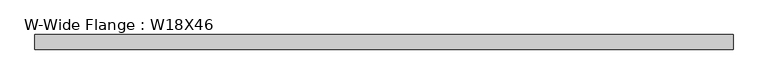
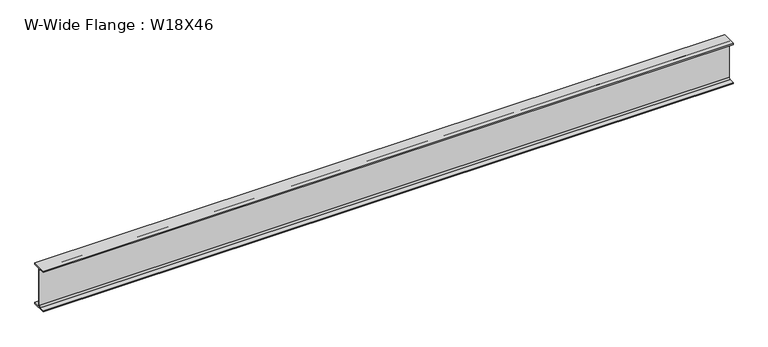
"""IFC4 building model written with IfcOpenShell, lengths in millimetres: beam geometry, W-Wide Flange : W18X46."""

from ifc_helpers import new_model, si_unit, point, frame, frame_2d, origin, place, context, project, spatial, polyline, circle_curve, trimmed, segment, composite_curve, outline, extrude, source, transform, mapped, element, save


def w_wide_flange_w18x46_b0132ec0(model_context):
    return source(origin(), model_context, "Body", "SweptSolid", [
        extrude(outline(composite_curve([segment(polyline([(76.962, -214.503), (76.962, -229.87), (-76.962, -229.87), (-76.962, -214.503), (-20.955, -214.503)]), True, "CONTINUOUS"), segment(trimmed(circle_curve(frame_2d((-20.955, -198.12)), 16.383), [point((-20.955, -214.503))], [point((-4.572, -198.12))], True, "CARTESIAN"), True, "CONTINUOUS"), segment(polyline([(-4.572, -198.12), (-4.572, 198.12)]), True, "CONTINUOUS"), segment(trimmed(circle_curve(frame_2d((-20.955, 198.12)), 16.383), [point((-4.572, 198.12))], [point((-20.955, 214.503))], True, "CARTESIAN"), True, "CONTINUOUS"), segment(polyline([(-20.955, 214.503), (-76.962, 214.503), (-76.962, 229.87), (76.962, 229.87), (76.962, 214.503), (20.955, 214.503)]), True, "CONTINUOUS"), segment(trimmed(circle_curve(frame_2d((20.955, 198.12)), 16.383), [point((20.955, 214.503))], [point((4.572, 198.12))], True, "CARTESIAN"), True, "CONTINUOUS"), segment(polyline([(4.572, 198.12), (4.572, -198.12)]), True, "CONTINUOUS"), segment(trimmed(circle_curve(frame_2d((20.955, -198.12)), 16.383), [point((4.572, -198.12))], [point((20.955, -214.503))], True, "CARTESIAN"), True, "CONTINUOUS"), segment(polyline([(20.955, -214.503), (76.962, -214.503)]), True, "CONTINUOUS")], self_intersect=False)), frame((-3648.0253906, 0.0, 0.0), z_axis=(1.0, 0.0, 0.0), x_axis=(0.0, 1.0, 0.0)), (0.0, 0.0, 1.0), 7358.7570312),
    ])


if __name__ == "__main__":
    model = new_model("IFC4")
    model_context = context("Model", 3, world=origin())
    ifc_project = project(units=[si_unit("LENGTHUNIT", "METRE", prefix="MILLI")], contexts=[model_context])
    site = spatial("IfcSite", under=ifc_project)
    building = spatial("IfcBuilding", under=site)
    placement = place(None, origin())
    w_wide_flange_w18x46_shape = w_wide_flange_w18x46_b0132ec0(model_context)
    element("IfcBeam", 1, ObjectType="W-Wide Flange : W18X46", at=placement, inside=building, context=model_context, shape_type="MappedRepresentation", body=[
        mapped(w_wide_flange_w18x46_shape, transform((0.0, 0.0, 0.0), x_axis=(1.0, 0.0, 0.0), y_axis=(0.0, 1.0, 0.0), z_axis=(0.0, 0.0, 1.0))),
    ])
    save(model, "model.ifc")

# Revit data of these elements
# Type "W-Wide Flange : W18X46"
#   Assembly Code = "B10"
#   W = 46
#   Length [instance default] = 1524 mm
#   bf = 153.924 mm
#   d = 459.74 mm
#   k = 31.75 mm
#   k2 = 16.383 mm
#   tf = 15.367 mm
#   tw = 9.144 mm
#   A = 0.00870966 m²
#   Structural Material [instance default] = Steel ASTM A992
# Element 1 (IfcBeam, "W-Wide Flange : W18X46")
#   Structural Material = Aluminum, Anodized Red
#   Materials on its faces: "Aluminum, Anodized Red"
# Materials
#   "Steel ASTM A992": class "Metal", colour RGB 128 0 0, transparency 0, Description = "Structural steel 50ksi", Cost = 0
#   "Aluminum, Anodized Red": class "Metal", colour RGB 120 120 120, transparency 0, Description = "Anodized aluminum, red", Cost = 0
